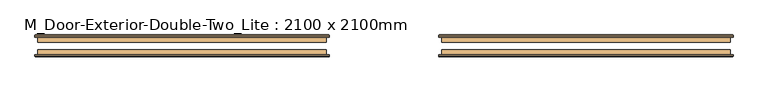
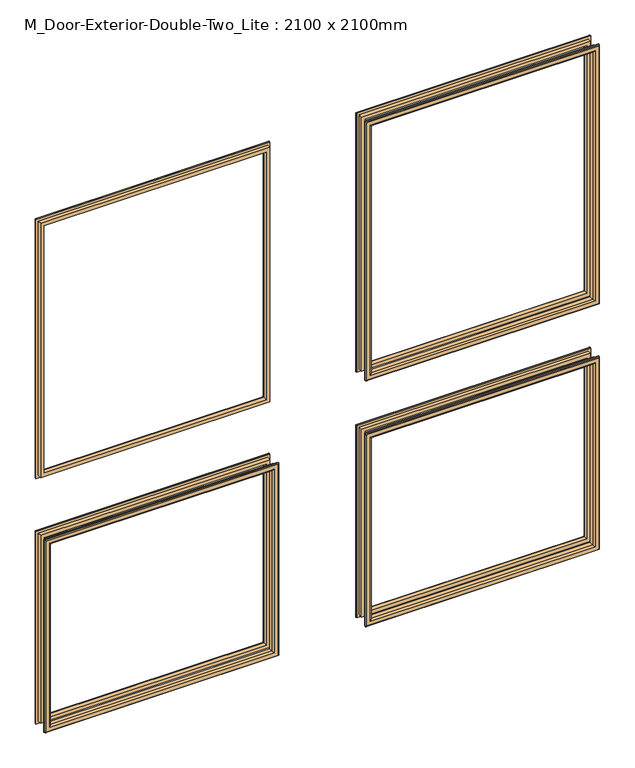
"""IFC4 building model written with IfcOpenShell, lengths in millimetres: door geometry, M_Door-Exterior-Double-Two_Lite : 2100 x 2100mm."""

from ifc_helpers import new_model, si_unit, frame, origin, place, context, project, spatial, ellipse_curve, source, transform, mapped, element, save
from ifc_brep_helpers import plane_surface, cylinder_surface, advanced_brep


def m_door_exterior_double_two_lite_2100_x_2100mm_e5180fcb(model_context):
    return source(origin(), model_context, "Body", "AdvancedBrep", [
        advanced_brep(
        [(-900.0, 31.35, 900.0), (-900.0, 43.85, 900.0), (-900.0, 43.85, 250.0), (-900.0, 31.35, 250.0), (-888.0, 44.85, 888.0), (-888.0, 31.35, 888.0), (-888.0, 31.35, 262.0), (-888.0, 44.85, 262.0), (-893.0, 49.85, 893.0), (-893.0, 49.85, 257.0), (-908.0, 47.85, 908.0), (-906.0, 49.85, 906.0), (-906.0, 49.85, 244.0), (-908.0, 47.85, 242.0), (-908.0, 43.85, 908.0), (-908.0, 43.85, 242.0), (-150.0, 43.85, 250.0), (-150.0, 31.35, 250.0), (-162.0, 31.35, 262.0), (-162.0, 44.85, 262.0), (-157.0, 49.85, 257.0), (-144.0, 49.85, 244.0), (-142.0, 47.85, 242.0), (-142.0, 43.85, 242.0), (-150.0, 43.85, 900.0), (-150.0, 31.35, 900.0), (-162.0, 31.35, 888.0), (-162.0, 44.85, 888.0), (-157.0, 49.85, 893.0), (-144.0, 49.85, 906.0), (-142.0, 47.85, 908.0), (-142.0, 43.85, 908.0)],
        [
            (0, 1),
            (1, 2),
            (2, 3),
            (3, 0),
            (4, 5),
            (5, 6),
            (6, 7),
            (7, 4),
            (8, 4, ellipse_curve(frame((-893.0, 44.85, 893.0), z_axis=(-0.7071067811865475, 0.0, -0.7071067811865475), x_axis=(-0.7071067811865474, 0.0, 0.7071067811865476)), 7.0710678, 5.0)),
            (7, 9, ellipse_curve(frame((-893.0, 44.85, 257.0), z_axis=(-0.7071067811865475, 0.0, 0.7071067811865475), x_axis=(0.7071067811865474, 0.0, 0.7071067811865476)), 7.0710678, 5.0)),
            (9, 8),
            (10, 11, ellipse_curve(frame((-906.0, 47.85, 906.0), z_axis=(-0.7071067811865475, 0.0, -0.7071067811865475), x_axis=(-0.7071067811865474, 0.0, 0.7071067811865476)), 2.8284271, 2.0)),
            (11, 12),
            (12, 13, ellipse_curve(frame((-906.0, 47.85, 244.0), z_axis=(-0.7071067811865475, 0.0, 0.7071067811865475), x_axis=(0.7071067811865474, 0.0, 0.7071067811865476)), 2.8284271, 2.0)),
            (13, 10),
            (14, 10),
            (13, 15),
            (15, 14),
            (2, 16),
            (16, 17),
            (17, 3),
            (6, 18),
            (18, 19),
            (19, 7),
            (19, 20, ellipse_curve(frame((-157.0, 44.85, 257.0), z_axis=(-0.7071067811865475, 0.0, -0.7071067811865475), x_axis=(-0.7071067811865476, 0.0, 0.7071067811865474)), 7.0710678, 5.0)),
            (20, 9),
            (12, 21),
            (21, 22, ellipse_curve(frame((-144.0, 47.85, 244.0), z_axis=(-0.7071067811865475, 0.0, -0.7071067811865475), x_axis=(-0.7071067811865476, 0.0, 0.7071067811865474)), 2.8284271, 2.0)),
            (22, 13),
            (22, 23),
            (23, 15),
            (16, 24),
            (24, 25),
            (25, 17),
            (18, 26),
            (26, 27),
            (27, 19),
            (27, 28, ellipse_curve(frame((-157.0, 44.85, 893.0), z_axis=(0.7071067811865475, 0.0, -0.7071067811865475), x_axis=(-0.7071067811865474, 0.0, -0.7071067811865476)), 7.0710678, 5.0)),
            (28, 20),
            (21, 29),
            (29, 30, ellipse_curve(frame((-144.0, 47.85, 906.0), z_axis=(0.7071067811865475, 0.0, -0.7071067811865475), x_axis=(-0.7071067811865474, 0.0, -0.7071067811865476)), 2.8284271, 2.0)),
            (30, 22),
            (30, 31),
            (31, 23),
            (31, 14),
            (1, 24),
            (0, 25),
            (5, 26),
            (4, 27),
            (8, 28),
            (11, 29),
            (10, 30),
        ],
        [
            plane_surface(frame((-900.0, 43.85, 900.0), z_axis=(-1.0, 0.0, 0.0), x_axis=(0.0, 0.0, -1.0))),
            plane_surface(frame((-888.0, 31.35, 888.0), z_axis=(1.0, 0.0, 0.0), x_axis=(0.0, 0.0, -1.0))),
            cylinder_surface(frame((-893.0, 44.85, 900.0), z_axis=(0.0, 0.0, 1.0), x_axis=(-1.0, 0.0, 0.0)), 5.0),
            cylinder_surface(frame((-906.0, 47.85, 900.0), z_axis=(0.0, 0.0, 1.0), x_axis=(-1.0, 0.0, 0.0)), 2.0),
            plane_surface(frame((-908.0, 47.85, 908.0), z_axis=(-1.0, 0.0, 0.0), x_axis=(0.0, 0.0, -1.0))),
            plane_surface(frame((-900.0, 43.85, 250.0), z_axis=(0.0, 0.0, -1.0), x_axis=(1.0, 0.0, 0.0))),
            plane_surface(frame((-888.0, 31.35, 262.0), z_axis=(0.0, 0.0, 1.0), x_axis=(1.0, 0.0, 0.0))),
            cylinder_surface(frame((-900.0, 44.85, 257.0), z_axis=(-1.0, 0.0, 0.0), x_axis=(0.0, 0.0, -1.0)), 5.0),
            cylinder_surface(frame((-900.0, 47.85, 244.0), z_axis=(-1.0, 0.0, 0.0), x_axis=(0.0, 0.0, -1.0)), 2.0),
            plane_surface(frame((-908.0, 47.85, 242.0), z_axis=(0.0, 0.0, -1.0), x_axis=(1.0, 0.0, 0.0))),
            plane_surface(frame((-150.0, 43.85, 250.0), z_axis=(1.0, 0.0, 0.0), x_axis=(0.0, 0.0, 1.0))),
            plane_surface(frame((-162.0, 31.35, 262.0), z_axis=(-1.0, 0.0, 0.0), x_axis=(0.0, 0.0, 1.0))),
            cylinder_surface(frame((-157.0, 44.85, 250.0), z_axis=(0.0, 0.0, -1.0), x_axis=(1.0, 0.0, 0.0)), 5.0),
            cylinder_surface(frame((-144.0, 47.85, 250.0), z_axis=(0.0, 0.0, -1.0), x_axis=(1.0, 0.0, 0.0)), 2.0),
            plane_surface(frame((-142.0, 47.85, 242.0), z_axis=(1.0, 0.0, 0.0), x_axis=(0.0, 0.0, 1.0))),
            plane_surface(frame((-142.0, 43.85, 908.0), z_axis=(0.0, -1.0, 0.0), x_axis=(-1.0, 0.0, 0.0))),
            plane_surface(frame((-150.0, 43.85, 900.0), z_axis=(0.0, 0.0, 1.0), x_axis=(-1.0, 0.0, 0.0))),
            plane_surface(frame((-150.0, 31.35, 900.0), z_axis=(0.0, -1.0, 0.0), x_axis=(-1.0, 0.0, 0.0))),
            plane_surface(frame((-162.0, 31.35, 888.0), z_axis=(0.0, 0.0, -1.0), x_axis=(-1.0, 0.0, 0.0))),
            cylinder_surface(frame((-150.0, 44.85, 893.0), z_axis=(1.0, 0.0, 0.0), x_axis=(0.0, 0.0, 1.0)), 5.0),
            plane_surface(frame((-157.0, 49.85, 893.0), z_axis=(0.0, 1.0, 0.0), x_axis=(-1.0, 0.0, 0.0))),
            cylinder_surface(frame((-150.0, 47.85, 906.0), z_axis=(1.0, 0.0, 0.0), x_axis=(0.0, 0.0, 1.0)), 2.0),
            plane_surface(frame((-142.0, 47.85, 908.0), z_axis=(0.0, 0.0, 1.0), x_axis=(-1.0, 0.0, 0.0))),
        ],
        [
            (0, [[1, 2, 3, 4]]),
            (1, [[5, 6, 7, 8]]),
            (2, [[9, -8, 10, 11]]),
            (3, [[12, 13, 14, 15]]),
            (4, [[16, -15, 17, 18]]),
            (5, [[-3, 19, 20, 21]]),
            (6, [[-7, 22, 23, 24]]),
            (7, [[-10, -24, 25, 26]]),
            (8, [[-14, 27, 28, 29]]),
            (9, [[-17, -29, 30, 31]]),
            (10, [[-20, 32, 33, 34]]),
            (11, [[-23, 35, 36, 37]]),
            (12, [[-25, -37, 38, 39]]),
            (13, [[-28, 40, 41, 42]]),
            (14, [[-30, -42, 43, 44]]),
            (15, [[-31, -44, 45, -18], [46, -32, -19, -2]]),
            (16, [[-33, -46, -1, 47]]),
            (17, [[-21, -34, -47, -4], [48, -35, -22, -6]]),
            (18, [[-36, -48, -5, 49]]),
            (19, [[-38, -49, -9, 50]]),
            (20, [[51, -40, -27, -13], [-26, -39, -50, -11]]),
            (21, [[-41, -51, -12, 52]]),
            (22, [[-43, -52, -16, -45]]),
        ],
    ),
        advanced_brep(
        [(150.0, 31.35, 900.0), (150.0, 43.85, 900.0), (150.0, 43.85, 250.0), (150.0, 31.35, 250.0), (162.0, 44.85, 888.0), (162.0, 31.35, 888.0), (162.0, 31.35, 262.0), (162.0, 44.85, 262.0), (157.0, 49.85, 893.0), (157.0, 49.85, 257.0), (142.0, 47.85, 908.0), (144.0, 49.85, 906.0), (144.0, 49.85, 244.0), (142.0, 47.85, 242.0), (142.0, 43.85, 908.0), (142.0, 43.85, 242.0), (900.0, 43.85, 250.0), (900.0, 31.35, 250.0), (888.0, 31.35, 262.0), (888.0, 44.85, 262.0), (893.0, 49.85, 257.0), (906.0, 49.85, 244.0), (908.0, 47.85, 242.0), (908.0, 43.85, 242.0), (900.0, 43.85, 900.0), (900.0, 31.35, 900.0), (888.0, 31.35, 888.0), (888.0, 44.85, 888.0), (893.0, 49.85, 893.0), (906.0, 49.85, 906.0), (908.0, 47.85, 908.0), (908.0, 43.85, 908.0)],
        [
            (0, 1),
            (1, 2),
            (2, 3),
            (3, 0),
            (4, 5),
            (5, 6),
            (6, 7),
            (7, 4),
            (8, 4, ellipse_curve(frame((157.0, 44.85, 893.0), z_axis=(-0.7071067811865475, 0.0, -0.7071067811865475), x_axis=(-0.7071067811865474, 0.0, 0.7071067811865476)), 7.0710678, 5.0)),
            (7, 9, ellipse_curve(frame((157.0, 44.85, 257.0), z_axis=(-0.7071067811865475, 0.0, 0.7071067811865475), x_axis=(0.7071067811865474, 0.0, 0.7071067811865476)), 7.0710678, 5.0)),
            (9, 8),
            (10, 11, ellipse_curve(frame((144.0, 47.85, 906.0), z_axis=(-0.7071067811865475, 0.0, -0.7071067811865475), x_axis=(-0.7071067811865474, 0.0, 0.7071067811865476)), 2.8284271, 2.0)),
            (11, 12),
            (12, 13, ellipse_curve(frame((144.0, 47.85, 244.0), z_axis=(-0.7071067811865475, 0.0, 0.7071067811865475), x_axis=(0.7071067811865474, 0.0, 0.7071067811865476)), 2.8284271, 2.0)),
            (13, 10),
            (14, 10),
            (13, 15),
            (15, 14),
            (2, 16),
            (16, 17),
            (17, 3),
            (6, 18),
            (18, 19),
            (19, 7),
            (19, 20, ellipse_curve(frame((893.0, 44.85, 257.0), z_axis=(-0.7071067811865475, 0.0, -0.7071067811865475), x_axis=(-0.7071067811865476, 0.0, 0.7071067811865474)), 7.0710678, 5.0)),
            (20, 9),
            (12, 21),
            (21, 22, ellipse_curve(frame((906.0, 47.85, 244.0), z_axis=(-0.7071067811865475, 0.0, -0.7071067811865475), x_axis=(-0.7071067811865476, 0.0, 0.7071067811865474)), 2.8284271, 2.0)),
            (22, 13),
            (22, 23),
            (23, 15),
            (16, 24),
            (24, 25),
            (25, 17),
            (18, 26),
            (26, 27),
            (27, 19),
            (27, 28, ellipse_curve(frame((893.0, 44.85, 893.0), z_axis=(0.7071067811865475, 0.0, -0.7071067811865475), x_axis=(-0.7071067811865474, 0.0, -0.7071067811865476)), 7.0710678, 5.0)),
            (28, 20),
            (21, 29),
            (29, 30, ellipse_curve(frame((906.0, 47.85, 906.0), z_axis=(0.7071067811865475, 0.0, -0.7071067811865475), x_axis=(-0.7071067811865474, 0.0, -0.7071067811865476)), 2.8284271, 2.0)),
            (30, 22),
            (30, 31),
            (31, 23),
            (31, 14),
            (1, 24),
            (0, 25),
            (5, 26),
            (4, 27),
            (8, 28),
            (11, 29),
            (10, 30),
        ],
        [
            plane_surface(frame((150.0, 43.85, 900.0), z_axis=(-1.0, 0.0, 0.0), x_axis=(0.0, 0.0, -1.0))),
            plane_surface(frame((162.0, 31.35, 888.0), z_axis=(1.0, 0.0, 0.0), x_axis=(0.0, 0.0, -1.0))),
            cylinder_surface(frame((157.0, 44.85, 900.0), z_axis=(0.0, 0.0, 1.0), x_axis=(-1.0, 0.0, 0.0)), 5.0),
            cylinder_surface(frame((144.0, 47.85, 900.0), z_axis=(0.0, 0.0, 1.0), x_axis=(-1.0, 0.0, 0.0)), 2.0),
            plane_surface(frame((142.0, 47.85, 908.0), z_axis=(-1.0, 0.0, 0.0), x_axis=(0.0, 0.0, -1.0))),
            plane_surface(frame((150.0, 43.85, 250.0), z_axis=(0.0, 0.0, -1.0), x_axis=(1.0, 0.0, 0.0))),
            plane_surface(frame((162.0, 31.35, 262.0), z_axis=(0.0, 0.0, 1.0), x_axis=(1.0, 0.0, 0.0))),
            cylinder_surface(frame((150.0, 44.85, 257.0), z_axis=(-1.0, 0.0, 0.0), x_axis=(0.0, 0.0, -1.0)), 5.0),
            cylinder_surface(frame((150.0, 47.85, 244.0), z_axis=(-1.0, 0.0, 0.0), x_axis=(0.0, 0.0, -1.0)), 2.0),
            plane_surface(frame((142.0, 47.85, 242.0), z_axis=(0.0, 0.0, -1.0), x_axis=(1.0, 0.0, 0.0))),
            plane_surface(frame((900.0, 43.85, 250.0), z_axis=(1.0, 0.0, 0.0), x_axis=(0.0, 0.0, 1.0))),
            plane_surface(frame((888.0, 31.35, 262.0), z_axis=(-1.0, 0.0, 0.0), x_axis=(0.0, 0.0, 1.0))),
            cylinder_surface(frame((893.0, 44.85, 250.0), z_axis=(0.0, 0.0, -1.0), x_axis=(1.0, 0.0, 0.0)), 5.0),
            cylinder_surface(frame((906.0, 47.85, 250.0), z_axis=(0.0, 0.0, -1.0), x_axis=(1.0, 0.0, 0.0)), 2.0),
            plane_surface(frame((908.0, 47.85, 242.0), z_axis=(1.0, 0.0, 0.0), x_axis=(0.0, 0.0, 1.0))),
            plane_surface(frame((908.0, 43.85, 908.0), z_axis=(0.0, -1.0, 0.0), x_axis=(-1.0, 0.0, 0.0))),
            plane_surface(frame((900.0, 43.85, 900.0), z_axis=(0.0, 0.0, 1.0), x_axis=(-1.0, 0.0, 0.0))),
            plane_surface(frame((900.0, 31.35, 900.0), z_axis=(0.0, -1.0, 0.0), x_axis=(-1.0, 0.0, 0.0))),
            plane_surface(frame((888.0, 31.35, 888.0), z_axis=(0.0, 0.0, -1.0), x_axis=(-1.0, 0.0, 0.0))),
            cylinder_surface(frame((900.0, 44.85, 893.0), z_axis=(1.0, 0.0, 0.0), x_axis=(0.0, 0.0, 1.0)), 5.0),
            plane_surface(frame((893.0, 49.85, 893.0), z_axis=(0.0, 1.0, 0.0), x_axis=(-1.0, 0.0, 0.0))),
            cylinder_surface(frame((900.0, 47.85, 906.0), z_axis=(1.0, 0.0, 0.0), x_axis=(0.0, 0.0, 1.0)), 2.0),
            plane_surface(frame((908.0, 47.85, 908.0), z_axis=(0.0, 0.0, 1.0), x_axis=(-1.0, 0.0, 0.0))),
        ],
        [
            (0, [[1, 2, 3, 4]]),
            (1, [[5, 6, 7, 8]]),
            (2, [[9, -8, 10, 11]]),
            (3, [[12, 13, 14, 15]]),
            (4, [[16, -15, 17, 18]]),
            (5, [[-3, 19, 20, 21]]),
            (6, [[-7, 22, 23, 24]]),
            (7, [[-10, -24, 25, 26]]),
            (8, [[-14, 27, 28, 29]]),
            (9, [[-17, -29, 30, 31]]),
            (10, [[-20, 32, 33, 34]]),
            (11, [[-23, 35, 36, 37]]),
            (12, [[-25, -37, 38, 39]]),
            (13, [[-28, 40, 41, 42]]),
            (14, [[-30, -42, 43, 44]]),
            (15, [[-31, -44, 45, -18], [46, -32, -19, -2]]),
            (16, [[-33, -46, -1, 47]]),
            (17, [[-21, -34, -47, -4], [48, -35, -22, -6]]),
            (18, [[-36, -48, -5, 49]]),
            (19, [[-38, -49, -9, 50]]),
            (20, [[51, -40, -27, -13], [-26, -39, -50, -11]]),
            (21, [[-41, -51, -12, 52]]),
            (22, [[-43, -52, -16, -45]]),
        ],
    ),
        advanced_brep(
        [(150.0, 31.35, 1980.0), (150.0, 43.85, 1980.0), (150.0, 43.85, 1100.0), (150.0, 31.35, 1100.0), (162.0, 44.85, 1968.0), (162.0, 31.35, 1968.0), (162.0, 31.35, 1112.0), (162.0, 44.85, 1112.0), (157.0, 49.85, 1973.0), (157.0, 49.85, 1107.0), (142.0, 47.85, 1988.0), (144.0, 49.85, 1986.0), (144.0, 49.85, 1094.0), (142.0, 47.85, 1092.0), (142.0, 43.85, 1988.0), (142.0, 43.85, 1092.0), (900.0, 43.85, 1100.0), (900.0, 31.35, 1100.0), (888.0, 31.35, 1112.0), (888.0, 44.85, 1112.0), (893.0, 49.85, 1107.0), (906.0, 49.85, 1094.0), (908.0, 47.85, 1092.0), (908.0, 43.85, 1092.0), (900.0, 43.85, 1980.0), (900.0, 31.35, 1980.0), (888.0, 31.35, 1968.0), (888.0, 44.85, 1968.0), (893.0, 49.85, 1973.0), (906.0, 49.85, 1986.0), (908.0, 47.85, 1988.0), (908.0, 43.85, 1988.0)],
        [
            (0, 1),
            (1, 2),
            (2, 3),
            (3, 0),
            (4, 5),
            (5, 6),
            (6, 7),
            (7, 4),
            (8, 4, ellipse_curve(frame((157.0, 44.85, 1973.0), z_axis=(-0.7071067811865475, 0.0, -0.7071067811865475), x_axis=(-0.7071067811865474, 0.0, 0.7071067811865476)), 7.0710678, 5.0)),
            (7, 9, ellipse_curve(frame((157.0, 44.85, 1107.0), z_axis=(-0.7071067811865475, 0.0, 0.7071067811865475), x_axis=(0.7071067811865474, 0.0, 0.7071067811865476)), 7.0710678, 5.0)),
            (9, 8),
            (10, 11, ellipse_curve(frame((144.0, 47.85, 1986.0), z_axis=(-0.7071067811865475, 0.0, -0.7071067811865475), x_axis=(-0.7071067811865474, 0.0, 0.7071067811865476)), 2.8284271, 2.0)),
            (11, 12),
            (12, 13, ellipse_curve(frame((144.0, 47.85, 1094.0), z_axis=(-0.7071067811865475, 0.0, 0.7071067811865475), x_axis=(0.7071067811865474, 0.0, 0.7071067811865476)), 2.8284271, 2.0)),
            (13, 10),
            (14, 10),
            (13, 15),
            (15, 14),
            (2, 16),
            (16, 17),
            (17, 3),
            (6, 18),
            (18, 19),
            (19, 7),
            (19, 20, ellipse_curve(frame((893.0, 44.85, 1107.0), z_axis=(-0.7071067811865475, 0.0, -0.7071067811865475), x_axis=(-0.7071067811865476, 0.0, 0.7071067811865474)), 7.0710678, 5.0)),
            (20, 9),
            (12, 21),
            (21, 22, ellipse_curve(frame((906.0, 47.85, 1094.0), z_axis=(-0.7071067811865475, 0.0, -0.7071067811865475), x_axis=(-0.7071067811865476, 0.0, 0.7071067811865474)), 2.8284271, 2.0)),
            (22, 13),
            (22, 23),
            (23, 15),
            (16, 24),
            (24, 25),
            (25, 17),
            (18, 26),
            (26, 27),
            (27, 19),
            (27, 28, ellipse_curve(frame((893.0, 44.85, 1973.0), z_axis=(0.7071067811865475, 0.0, -0.7071067811865475), x_axis=(-0.7071067811865474, 0.0, -0.7071067811865476)), 7.0710678, 5.0)),
            (28, 20),
            (21, 29),
            (29, 30, ellipse_curve(frame((906.0, 47.85, 1986.0), z_axis=(0.7071067811865475, 0.0, -0.7071067811865475), x_axis=(-0.7071067811865474, 0.0, -0.7071067811865476)), 2.8284271, 2.0)),
            (30, 22),
            (30, 31),
            (31, 23),
            (31, 14),
            (1, 24),
            (0, 25),
            (5, 26),
            (4, 27),
            (8, 28),
            (11, 29),
            (10, 30),
        ],
        [
            plane_surface(frame((150.0, 43.85, 1980.0), z_axis=(-1.0, 0.0, 0.0), x_axis=(0.0, 0.0, -1.0))),
            plane_surface(frame((162.0, 31.35, 1968.0), z_axis=(1.0, 0.0, 0.0), x_axis=(0.0, 0.0, -1.0))),
            cylinder_surface(frame((157.0, 44.85, 1980.0), z_axis=(0.0, 0.0, 1.0), x_axis=(-1.0, 0.0, 0.0)), 5.0),
            cylinder_surface(frame((144.0, 47.85, 1980.0), z_axis=(0.0, 0.0, 1.0), x_axis=(-1.0, 0.0, 0.0)), 2.0),
            plane_surface(frame((142.0, 47.85, 1988.0), z_axis=(-1.0, 0.0, 0.0), x_axis=(0.0, 0.0, -1.0))),
            plane_surface(frame((150.0, 43.85, 1100.0), z_axis=(0.0, 0.0, -1.0), x_axis=(1.0, 0.0, 0.0))),
            plane_surface(frame((162.0, 31.35, 1112.0), z_axis=(0.0, 0.0, 1.0), x_axis=(1.0, 0.0, 0.0))),
            cylinder_surface(frame((150.0, 44.85, 1107.0), z_axis=(-1.0, 0.0, 0.0), x_axis=(0.0, 0.0, -1.0)), 5.0),
            cylinder_surface(frame((150.0, 47.85, 1094.0), z_axis=(-1.0, 0.0, 0.0), x_axis=(0.0, 0.0, -1.0)), 2.0),
            plane_surface(frame((142.0, 47.85, 1092.0), z_axis=(0.0, 0.0, -1.0), x_axis=(1.0, 0.0, 0.0))),
            plane_surface(frame((900.0, 43.85, 1100.0), z_axis=(1.0, 0.0, 0.0), x_axis=(0.0, 0.0, 1.0))),
            plane_surface(frame((888.0, 31.35, 1112.0), z_axis=(-1.0, 0.0, 0.0), x_axis=(0.0, 0.0, 1.0))),
            cylinder_surface(frame((893.0, 44.85, 1100.0), z_axis=(0.0, 0.0, -1.0), x_axis=(1.0, 0.0, 0.0)), 5.0),
            cylinder_surface(frame((906.0, 47.85, 1100.0), z_axis=(0.0, 0.0, -1.0), x_axis=(1.0, 0.0, 0.0)), 2.0),
            plane_surface(frame((908.0, 47.85, 1092.0), z_axis=(1.0, 0.0, 0.0), x_axis=(0.0, 0.0, 1.0))),
            plane_surface(frame((908.0, 43.85, 1988.0), z_axis=(0.0, -1.0, 0.0), x_axis=(-1.0, 0.0, 0.0))),
            plane_surface(frame((900.0, 43.85, 1980.0), z_axis=(0.0, 0.0, 1.0), x_axis=(-1.0, 0.0, 0.0))),
            plane_surface(frame((900.0, 31.35, 1980.0), z_axis=(0.0, -1.0, 0.0), x_axis=(-1.0, 0.0, 0.0))),
            plane_surface(frame((888.0, 31.35, 1968.0), z_axis=(0.0, 0.0, -1.0), x_axis=(-1.0, 0.0, 0.0))),
            cylinder_surface(frame((900.0, 44.85, 1973.0), z_axis=(1.0, 0.0, 0.0), x_axis=(0.0, 0.0, 1.0)), 5.0),
            plane_surface(frame((893.0, 49.85, 1973.0), z_axis=(0.0, 1.0, 0.0), x_axis=(-1.0, 0.0, 0.0))),
            cylinder_surface(frame((900.0, 47.85, 1986.0), z_axis=(1.0, 0.0, 0.0), x_axis=(0.0, 0.0, 1.0)), 2.0),
            plane_surface(frame((908.0, 47.85, 1988.0), z_axis=(0.0, 0.0, 1.0), x_axis=(-1.0, 0.0, 0.0))),
        ],
        [
            (0, [[1, 2, 3, 4]]),
            (1, [[5, 6, 7, 8]]),
            (2, [[9, -8, 10, 11]]),
            (3, [[12, 13, 14, 15]]),
            (4, [[16, -15, 17, 18]]),
            (5, [[-3, 19, 20, 21]]),
            (6, [[-7, 22, 23, 24]]),
            (7, [[-10, -24, 25, 26]]),
            (8, [[-14, 27, 28, 29]]),
            (9, [[-17, -29, 30, 31]]),
            (10, [[-20, 32, 33, 34]]),
            (11, [[-23, 35, 36, 37]]),
            (12, [[-25, -37, 38, 39]]),
            (13, [[-28, 40, 41, 42]]),
            (14, [[-30, -42, 43, 44]]),
            (15, [[-31, -44, 45, -18], [46, -32, -19, -2]]),
            (16, [[-33, -46, -1, 47]]),
            (17, [[-21, -34, -47, -4], [48, -35, -22, -6]]),
            (18, [[-36, -48, -5, 49]]),
            (19, [[-38, -49, -9, 50]]),
            (20, [[51, -40, -27, -13], [-26, -39, -50, -11]]),
            (21, [[-41, -51, -12, 52]]),
            (22, [[-43, -52, -16, -45]]),
        ],
    ),
        advanced_brep(
        [(-900.0, 31.35, 1980.0), (-900.0, 43.85, 1980.0), (-900.0, 43.85, 1100.0), (-900.0, 31.35, 1100.0), (-888.0, 44.85, 1968.0), (-888.0, 31.35, 1968.0), (-888.0, 31.35, 1112.0), (-888.0, 44.85, 1112.0), (-893.0, 49.85, 1973.0), (-893.0, 49.85, 1107.0), (-908.0, 47.85, 1988.0), (-906.0, 49.85, 1986.0), (-906.0, 49.85, 1094.0), (-908.0, 47.85, 1092.0), (-908.0, 43.85, 1988.0), (-908.0, 43.85, 1092.0), (-150.0, 43.85, 1100.0), (-150.0, 31.35, 1100.0), (-162.0, 31.35, 1112.0), (-162.0, 44.85, 1112.0), (-157.0, 49.85, 1107.0), (-144.0, 49.85, 1094.0), (-142.0, 47.85, 1092.0), (-142.0, 43.85, 1092.0), (-150.0, 43.85, 1980.0), (-150.0, 31.35, 1980.0), (-162.0, 31.35, 1968.0), (-162.0, 44.85, 1968.0), (-157.0, 49.85, 1973.0), (-144.0, 49.85, 1986.0), (-142.0, 47.85, 1988.0), (-142.0, 43.85, 1988.0)],
        [
            (0, 1),
            (1, 2),
            (2, 3),
            (3, 0),
            (4, 5),
            (5, 6),
            (6, 7),
            (7, 4),
            (8, 4, ellipse_curve(frame((-893.0, 44.85, 1973.0), z_axis=(-0.7071067811865475, 0.0, -0.7071067811865475), x_axis=(-0.7071067811865474, 0.0, 0.7071067811865476)), 7.0710678, 5.0)),
            (7, 9, ellipse_curve(frame((-893.0, 44.85, 1107.0), z_axis=(-0.7071067811865475, 0.0, 0.7071067811865475), x_axis=(0.7071067811865474, 0.0, 0.7071067811865476)), 7.0710678, 5.0)),
            (9, 8),
            (10, 11, ellipse_curve(frame((-906.0, 47.85, 1986.0), z_axis=(-0.7071067811865475, 0.0, -0.7071067811865475), x_axis=(-0.7071067811865474, 0.0, 0.7071067811865476)), 2.8284271, 2.0)),
            (11, 12),
            (12, 13, ellipse_curve(frame((-906.0, 47.85, 1094.0), z_axis=(-0.7071067811865475, 0.0, 0.7071067811865475), x_axis=(0.7071067811865474, 0.0, 0.7071067811865476)), 2.8284271, 2.0)),
            (13, 10),
            (14, 10),
            (13, 15),
            (15, 14),
            (2, 16),
            (16, 17),
            (17, 3),
            (6, 18),
            (18, 19),
            (19, 7),
            (19, 20, ellipse_curve(frame((-157.0, 44.85, 1107.0), z_axis=(-0.7071067811865475, 0.0, -0.7071067811865475), x_axis=(-0.7071067811865476, 0.0, 0.7071067811865474)), 7.0710678, 5.0)),
            (20, 9),
            (12, 21),
            (21, 22, ellipse_curve(frame((-144.0, 47.85, 1094.0), z_axis=(-0.7071067811865475, 0.0, -0.7071067811865475), x_axis=(-0.7071067811865476, 0.0, 0.7071067811865474)), 2.8284271, 2.0)),
            (22, 13),
            (22, 23),
            (23, 15),
            (16, 24),
            (24, 25),
            (25, 17),
            (18, 26),
            (26, 27),
            (27, 19),
            (27, 28, ellipse_curve(frame((-157.0, 44.85, 1973.0), z_axis=(0.7071067811865475, 0.0, -0.7071067811865475), x_axis=(-0.7071067811865474, 0.0, -0.7071067811865476)), 7.0710678, 5.0)),
            (28, 20),
            (21, 29),
            (29, 30, ellipse_curve(frame((-144.0, 47.85, 1986.0), z_axis=(0.7071067811865475, 0.0, -0.7071067811865475), x_axis=(-0.7071067811865474, 0.0, -0.7071067811865476)), 2.8284271, 2.0)),
            (30, 22),
            (30, 31),
            (31, 23),
            (31, 14),
            (1, 24),
            (0, 25),
            (5, 26),
            (4, 27),
            (8, 28),
            (11, 29),
            (10, 30),
        ],
        [
            plane_surface(frame((-900.0, 43.85, 1980.0), z_axis=(-1.0, 0.0, 0.0), x_axis=(0.0, 0.0, -1.0))),
            plane_surface(frame((-888.0, 31.35, 1968.0), z_axis=(1.0, 0.0, 0.0), x_axis=(0.0, 0.0, -1.0))),
            cylinder_surface(frame((-893.0, 44.85, 1980.0), z_axis=(0.0, 0.0, 1.0), x_axis=(-1.0, 0.0, 0.0)), 5.0),
            cylinder_surface(frame((-906.0, 47.85, 1980.0), z_axis=(0.0, 0.0, 1.0), x_axis=(-1.0, 0.0, 0.0)), 2.0),
            plane_surface(frame((-908.0, 47.85, 1988.0), z_axis=(-1.0, 0.0, 0.0), x_axis=(0.0, 0.0, -1.0))),
            plane_surface(frame((-900.0, 43.85, 1100.0), z_axis=(0.0, 0.0, -1.0), x_axis=(1.0, 0.0, 0.0))),
            plane_surface(frame((-888.0, 31.35, 1112.0), z_axis=(0.0, 0.0, 1.0), x_axis=(1.0, 0.0, 0.0))),
            cylinder_surface(frame((-900.0, 44.85, 1107.0), z_axis=(-1.0, 0.0, 0.0), x_axis=(0.0, 0.0, -1.0)), 5.0),
            cylinder_surface(frame((-900.0, 47.85, 1094.0), z_axis=(-1.0, 0.0, 0.0), x_axis=(0.0, 0.0, -1.0)), 2.0),
            plane_surface(frame((-908.0, 47.85, 1092.0), z_axis=(0.0, 0.0, -1.0), x_axis=(1.0, 0.0, 0.0))),
            plane_surface(frame((-150.0, 43.85, 1100.0), z_axis=(1.0, 0.0, 0.0), x_axis=(0.0, 0.0, 1.0))),
            plane_surface(frame((-162.0, 31.35, 1112.0), z_axis=(-1.0, 0.0, 0.0), x_axis=(0.0, 0.0, 1.0))),
            cylinder_surface(frame((-157.0, 44.85, 1100.0), z_axis=(0.0, 0.0, -1.0), x_axis=(1.0, 0.0, 0.0)), 5.0),
            cylinder_surface(frame((-144.0, 47.85, 1100.0), z_axis=(0.0, 0.0, -1.0), x_axis=(1.0, 0.0, 0.0)), 2.0),
            plane_surface(frame((-142.0, 47.85, 1092.0), z_axis=(1.0, 0.0, 0.0), x_axis=(0.0, 0.0, 1.0))),
            plane_surface(frame((-142.0, 43.85, 1988.0), z_axis=(0.0, -1.0, 0.0), x_axis=(-1.0, 0.0, 0.0))),
            plane_surface(frame((-150.0, 43.85, 1980.0), z_axis=(0.0, 0.0, 1.0), x_axis=(-1.0, 0.0, 0.0))),
            plane_surface(frame((-150.0, 31.35, 1980.0), z_axis=(0.0, -1.0, 0.0), x_axis=(-1.0, 0.0, 0.0))),
            plane_surface(frame((-162.0, 31.35, 1968.0), z_axis=(0.0, 0.0, -1.0), x_axis=(-1.0, 0.0, 0.0))),
            cylinder_surface(frame((-150.0, 44.85, 1973.0), z_axis=(1.0, 0.0, 0.0), x_axis=(0.0, 0.0, 1.0)), 5.0),
            plane_surface(frame((-157.0, 49.85, 1973.0), z_axis=(0.0, 1.0, 0.0), x_axis=(-1.0, 0.0, 0.0))),
            cylinder_surface(frame((-150.0, 47.85, 1986.0), z_axis=(1.0, 0.0, 0.0), x_axis=(0.0, 0.0, 1.0)), 2.0),
            plane_surface(frame((-142.0, 47.85, 1988.0), z_axis=(0.0, 0.0, 1.0), x_axis=(-1.0, 0.0, 0.0))),
        ],
        [
            (0, [[1, 2, 3, 4]]),
            (1, [[5, 6, 7, 8]]),
            (2, [[9, -8, 10, 11]]),
            (3, [[12, 13, 14, 15]]),
            (4, [[16, -15, 17, 18]]),
            (5, [[-3, 19, 20, 21]]),
            (6, [[-7, 22, 23, 24]]),
            (7, [[-10, -24, 25, 26]]),
            (8, [[-14, 27, 28, 29]]),
            (9, [[-17, -29, 30, 31]]),
            (10, [[-20, 32, 33, 34]]),
            (11, [[-23, 35, 36, 37]]),
            (12, [[-25, -37, 38, 39]]),
            (13, [[-28, 40, 41, 42]]),
            (14, [[-30, -42, 43, 44]]),
            (15, [[-31, -44, 45, -18], [46, -32, -19, -2]]),
            (16, [[-33, -46, -1, 47]]),
            (17, [[-21, -34, -47, -4], [48, -35, -22, -6]]),
            (18, [[-36, -48, -5, 49]]),
            (19, [[-38, -49, -9, 50]]),
            (20, [[51, -40, -27, -13], [-26, -39, -50, -11]]),
            (21, [[-41, -51, -12, 52]]),
            (22, [[-43, -52, -16, -45]]),
        ],
    ),
        advanced_brep(
        [(-900.0, 11.35, 250.0), (-900.0, -1.15, 250.0), (-900.0, -1.15, 900.0), (-900.0, 11.35, 900.0), (-888.0, -2.15, 262.0), (-888.0, 11.35, 262.0), (-888.0, 11.35, 888.0), (-888.0, -2.15, 888.0), (-893.0, -7.15, 257.0), (-893.0, -7.15, 893.0), (-908.0, -5.15, 242.0), (-906.0, -7.15, 244.0), (-906.0, -7.15, 906.0), (-908.0, -5.15, 908.0), (-908.0, -1.15, 242.0), (-908.0, -1.15, 908.0), (-150.0, -1.15, 900.0), (-150.0, 11.35, 900.0), (-162.0, 11.35, 888.0), (-162.0, -2.15, 888.0), (-157.0, -7.15, 893.0), (-144.0, -7.15, 906.0), (-142.0, -5.15, 908.0), (-142.0, -1.15, 908.0), (-150.0, -1.15, 250.0), (-150.0, 11.35, 250.0), (-162.0, 11.35, 262.0), (-162.0, -2.15, 262.0), (-157.0, -7.15, 257.0), (-144.0, -7.15, 244.0), (-142.0, -5.15, 242.0), (-142.0, -1.15, 242.0)],
        [
            (0, 1),
            (1, 2),
            (2, 3),
            (3, 0),
            (4, 5),
            (5, 6),
            (6, 7),
            (7, 4),
            (8, 4, ellipse_curve(frame((-893.0, -2.15, 257.0), z_axis=(-0.7071067811865475, 0.0, 0.7071067811865475), x_axis=(-0.7071067811865474, 0.0, -0.7071067811865476)), 7.0710678, 5.0)),
            (7, 9, ellipse_curve(frame((-893.0, -2.15, 893.0), z_axis=(-0.7071067811865475, 0.0, -0.7071067811865475), x_axis=(0.7071067811865474, 0.0, -0.7071067811865476)), 7.0710678, 5.0)),
            (9, 8),
            (10, 11, ellipse_curve(frame((-906.0, -5.15, 244.0), z_axis=(-0.7071067811865475, 0.0, 0.7071067811865475), x_axis=(-0.7071067811865474, 0.0, -0.7071067811865476)), 2.8284271, 2.0)),
            (11, 12),
            (12, 13, ellipse_curve(frame((-906.0, -5.15, 906.0), z_axis=(-0.7071067811865475, 0.0, -0.7071067811865475), x_axis=(0.7071067811865474, 0.0, -0.7071067811865476)), 2.8284271, 2.0)),
            (13, 10),
            (14, 10),
            (13, 15),
            (15, 14),
            (2, 16),
            (16, 17),
            (17, 3),
            (6, 18),
            (18, 19),
            (19, 7),
            (19, 20, ellipse_curve(frame((-157.0, -2.15, 893.0), z_axis=(-0.7071067811865475, 0.0, 0.7071067811865475), x_axis=(-0.7071067811865476, 0.0, -0.7071067811865474)), 7.0710678, 5.0)),
            (20, 9),
            (12, 21),
            (21, 22, ellipse_curve(frame((-144.0, -5.15, 906.0), z_axis=(-0.7071067811865475, 0.0, 0.7071067811865475), x_axis=(-0.7071067811865476, 0.0, -0.7071067811865474)), 2.8284271, 2.0)),
            (22, 13),
            (22, 23),
            (23, 15),
            (16, 24),
            (24, 25),
            (25, 17),
            (18, 26),
            (26, 27),
            (27, 19),
            (27, 28, ellipse_curve(frame((-157.0, -2.15, 257.0), z_axis=(0.7071067811865475, 0.0, 0.7071067811865475), x_axis=(-0.7071067811865474, 0.0, 0.7071067811865476)), 7.0710678, 5.0)),
            (28, 20),
            (21, 29),
            (29, 30, ellipse_curve(frame((-144.0, -5.15, 244.0), z_axis=(0.7071067811865475, 0.0, 0.7071067811865475), x_axis=(-0.7071067811865474, 0.0, 0.7071067811865476)), 2.8284271, 2.0)),
            (30, 22),
            (30, 31),
            (31, 23),
            (31, 14),
            (1, 24),
            (0, 25),
            (5, 26),
            (4, 27),
            (8, 28),
            (11, 29),
            (10, 30),
        ],
        [
            plane_surface(frame((-900.0, -1.15, 250.0), z_axis=(-1.0, 0.0, 0.0), x_axis=(0.0, 0.0, 1.0))),
            plane_surface(frame((-888.0, 11.35, 262.0), z_axis=(1.0, 0.0, 0.0), x_axis=(0.0, 0.0, 1.0))),
            cylinder_surface(frame((-893.0, -2.15, 250.0), z_axis=(0.0, 0.0, -1.0), x_axis=(-1.0, 0.0, 0.0)), 5.0),
            cylinder_surface(frame((-906.0, -5.15, 250.0), z_axis=(0.0, 0.0, -1.0), x_axis=(-1.0, 0.0, 0.0)), 2.0),
            plane_surface(frame((-908.0, -5.15, 242.0), z_axis=(-1.0, 0.0, 0.0), x_axis=(0.0, 0.0, 1.0))),
            plane_surface(frame((-900.0, -1.15, 900.0), z_axis=(0.0, 0.0, 1.0), x_axis=(1.0, 0.0, 0.0))),
            plane_surface(frame((-888.0, 11.35, 888.0), z_axis=(0.0, 0.0, -1.0), x_axis=(1.0, 0.0, 0.0))),
            cylinder_surface(frame((-900.0, -2.15, 893.0), z_axis=(-1.0, 0.0, 0.0), x_axis=(0.0, 0.0, 1.0)), 5.0),
            cylinder_surface(frame((-900.0, -5.15, 906.0), z_axis=(-1.0, 0.0, 0.0), x_axis=(0.0, 0.0, 1.0)), 2.0),
            plane_surface(frame((-908.0, -5.15, 908.0), z_axis=(0.0, 0.0, 1.0), x_axis=(1.0, 0.0, 0.0))),
            plane_surface(frame((-150.0, -1.15, 900.0), z_axis=(1.0, 0.0, 0.0), x_axis=(0.0, 0.0, -1.0))),
            plane_surface(frame((-162.0, 11.35, 888.0), z_axis=(-1.0, 0.0, 0.0), x_axis=(0.0, 0.0, -1.0))),
            cylinder_surface(frame((-157.0, -2.15, 900.0), z_axis=(0.0, 0.0, 1.0), x_axis=(1.0, 0.0, 0.0)), 5.0),
            cylinder_surface(frame((-144.0, -5.15, 900.0), z_axis=(0.0, 0.0, 1.0), x_axis=(1.0, 0.0, 0.0)), 2.0),
            plane_surface(frame((-142.0, -5.15, 908.0), z_axis=(1.0, 0.0, 0.0), x_axis=(0.0, 0.0, -1.0))),
            plane_surface(frame((-142.0, -1.15, 242.0), z_axis=(0.0, 1.0, 0.0), x_axis=(-1.0, 0.0, 0.0))),
            plane_surface(frame((-150.0, -1.15, 250.0), z_axis=(0.0, 0.0, -1.0), x_axis=(-1.0, 0.0, 0.0))),
            plane_surface(frame((-150.0, 11.35, 250.0), z_axis=(0.0, 1.0, 0.0), x_axis=(-1.0, 0.0, 0.0))),
            plane_surface(frame((-162.0, 11.35, 262.0), z_axis=(0.0, 0.0, 1.0), x_axis=(-1.0, 0.0, 0.0))),
            cylinder_surface(frame((-150.0, -2.15, 257.0), z_axis=(1.0, 0.0, 0.0), x_axis=(0.0, 0.0, -1.0)), 5.0),
            plane_surface(frame((-157.0, -7.15, 257.0), z_axis=(0.0, -1.0, 0.0), x_axis=(-1.0, 0.0, 0.0))),
            cylinder_surface(frame((-150.0, -5.15, 244.0), z_axis=(1.0, 0.0, 0.0), x_axis=(0.0, 0.0, -1.0)), 2.0),
            plane_surface(frame((-142.0, -5.15, 242.0), z_axis=(0.0, 0.0, -1.0), x_axis=(-1.0, 0.0, 0.0))),
        ],
        [
            (0, [[1, 2, 3, 4]]),
            (1, [[5, 6, 7, 8]]),
            (2, [[9, -8, 10, 11]]),
            (3, [[12, 13, 14, 15]]),
            (4, [[16, -15, 17, 18]]),
            (5, [[-3, 19, 20, 21]]),
            (6, [[-7, 22, 23, 24]]),
            (7, [[-10, -24, 25, 26]]),
            (8, [[-14, 27, 28, 29]]),
            (9, [[-17, -29, 30, 31]]),
            (10, [[-20, 32, 33, 34]]),
            (11, [[-23, 35, 36, 37]]),
            (12, [[-25, -37, 38, 39]]),
            (13, [[-28, 40, 41, 42]]),
            (14, [[-30, -42, 43, 44]]),
            (15, [[-31, -44, 45, -18], [46, -32, -19, -2]]),
            (16, [[-33, -46, -1, 47]]),
            (17, [[-21, -34, -47, -4], [48, -35, -22, -6]]),
            (18, [[-36, -48, -5, 49]]),
            (19, [[-38, -49, -9, 50]]),
            (20, [[51, -40, -27, -13], [-26, -39, -50, -11]]),
            (21, [[-41, -51, -12, 52]]),
            (22, [[-43, -52, -16, -45]]),
        ],
    ),
        advanced_brep(
        [(150.0, 11.35, 250.0), (150.0, -1.15, 250.0), (150.0, -1.15, 900.0), (150.0, 11.35, 900.0), (162.0, -2.15, 262.0), (162.0, 11.35, 262.0), (162.0, 11.35, 888.0), (162.0, -2.15, 888.0), (157.0, -7.15, 257.0), (157.0, -7.15, 893.0), (142.0, -5.15, 242.0), (144.0, -7.15, 244.0), (144.0, -7.15, 906.0), (142.0, -5.15, 908.0), (142.0, -1.15, 242.0), (142.0, -1.15, 908.0), (900.0, -1.15, 900.0), (900.0, 11.35, 900.0), (888.0, 11.35, 888.0), (888.0, -2.15, 888.0), (893.0, -7.15, 893.0), (906.0, -7.15, 906.0), (908.0, -5.15, 908.0), (908.0, -1.15, 908.0), (900.0, -1.15, 250.0), (900.0, 11.35, 250.0), (888.0, 11.35, 262.0), (888.0, -2.15, 262.0), (893.0, -7.15, 257.0), (906.0, -7.15, 244.0), (908.0, -5.15, 242.0), (908.0, -1.15, 242.0)],
        [
            (0, 1),
            (1, 2),
            (2, 3),
            (3, 0),
            (4, 5),
            (5, 6),
            (6, 7),
            (7, 4),
            (8, 4, ellipse_curve(frame((157.0, -2.15, 257.0), z_axis=(-0.7071067811865475, 0.0, 0.7071067811865475), x_axis=(-0.7071067811865474, 0.0, -0.7071067811865476)), 7.0710678, 5.0)),
            (7, 9, ellipse_curve(frame((157.0, -2.15, 893.0), z_axis=(-0.7071067811865475, 0.0, -0.7071067811865475), x_axis=(0.7071067811865474, 0.0, -0.7071067811865476)), 7.0710678, 5.0)),
            (9, 8),
            (10, 11, ellipse_curve(frame((144.0, -5.15, 244.0), z_axis=(-0.7071067811865475, 0.0, 0.7071067811865475), x_axis=(-0.7071067811865474, 0.0, -0.7071067811865476)), 2.8284271, 2.0)),
            (11, 12),
            (12, 13, ellipse_curve(frame((144.0, -5.15, 906.0), z_axis=(-0.7071067811865475, 0.0, -0.7071067811865475), x_axis=(0.7071067811865474, 0.0, -0.7071067811865476)), 2.8284271, 2.0)),
            (13, 10),
            (14, 10),
            (13, 15),
            (15, 14),
            (2, 16),
            (16, 17),
            (17, 3),
            (6, 18),
            (18, 19),
            (19, 7),
            (19, 20, ellipse_curve(frame((893.0, -2.15, 893.0), z_axis=(-0.7071067811865475, 0.0, 0.7071067811865475), x_axis=(-0.7071067811865476, 0.0, -0.7071067811865474)), 7.0710678, 5.0)),
            (20, 9),
            (12, 21),
            (21, 22, ellipse_curve(frame((906.0, -5.15, 906.0), z_axis=(-0.7071067811865475, 0.0, 0.7071067811865475), x_axis=(-0.7071067811865476, 0.0, -0.7071067811865474)), 2.8284271, 2.0)),
            (22, 13),
            (22, 23),
            (23, 15),
            (16, 24),
            (24, 25),
            (25, 17),
            (18, 26),
            (26, 27),
            (27, 19),
            (27, 28, ellipse_curve(frame((893.0, -2.15, 257.0), z_axis=(0.7071067811865475, 0.0, 0.7071067811865475), x_axis=(-0.7071067811865474, 0.0, 0.7071067811865476)), 7.0710678, 5.0)),
            (28, 20),
            (21, 29),
            (29, 30, ellipse_curve(frame((906.0, -5.15, 244.0), z_axis=(0.7071067811865475, 0.0, 0.7071067811865475), x_axis=(-0.7071067811865474, 0.0, 0.7071067811865476)), 2.8284271, 2.0)),
            (30, 22),
            (30, 31),
            (31, 23),
            (31, 14),
            (1, 24),
            (0, 25),
            (5, 26),
            (4, 27),
            (8, 28),
            (11, 29),
            (10, 30),
        ],
        [
            plane_surface(frame((150.0, -1.15, 250.0), z_axis=(-1.0, 0.0, 0.0), x_axis=(0.0, 0.0, 1.0))),
            plane_surface(frame((162.0, 11.35, 262.0), z_axis=(1.0, 0.0, 0.0), x_axis=(0.0, 0.0, 1.0))),
            cylinder_surface(frame((157.0, -2.15, 250.0), z_axis=(0.0, 0.0, -1.0), x_axis=(-1.0, 0.0, 0.0)), 5.0),
            cylinder_surface(frame((144.0, -5.15, 250.0), z_axis=(0.0, 0.0, -1.0), x_axis=(-1.0, 0.0, 0.0)), 2.0),
            plane_surface(frame((142.0, -5.15, 242.0), z_axis=(-1.0, 0.0, 0.0), x_axis=(0.0, 0.0, 1.0))),
            plane_surface(frame((150.0, -1.15, 900.0), z_axis=(0.0, 0.0, 1.0), x_axis=(1.0, 0.0, 0.0))),
            plane_surface(frame((162.0, 11.35, 888.0), z_axis=(0.0, 0.0, -1.0), x_axis=(1.0, 0.0, 0.0))),
            cylinder_surface(frame((150.0, -2.15, 893.0), z_axis=(-1.0, 0.0, 0.0), x_axis=(0.0, 0.0, 1.0)), 5.0),
            cylinder_surface(frame((150.0, -5.15, 906.0), z_axis=(-1.0, 0.0, 0.0), x_axis=(0.0, 0.0, 1.0)), 2.0),
            plane_surface(frame((142.0, -5.15, 908.0), z_axis=(0.0, 0.0, 1.0), x_axis=(1.0, 0.0, 0.0))),
            plane_surface(frame((900.0, -1.15, 900.0), z_axis=(1.0, 0.0, 0.0), x_axis=(0.0, 0.0, -1.0))),
            plane_surface(frame((888.0, 11.35, 888.0), z_axis=(-1.0, 0.0, 0.0), x_axis=(0.0, 0.0, -1.0))),
            cylinder_surface(frame((893.0, -2.15, 900.0), z_axis=(0.0, 0.0, 1.0), x_axis=(1.0, 0.0, 0.0)), 5.0),
            cylinder_surface(frame((906.0, -5.15, 900.0), z_axis=(0.0, 0.0, 1.0), x_axis=(1.0, 0.0, 0.0)), 2.0),
            plane_surface(frame((908.0, -5.15, 908.0), z_axis=(1.0, 0.0, 0.0), x_axis=(0.0, 0.0, -1.0))),
            plane_surface(frame((908.0, -1.15, 242.0), z_axis=(0.0, 1.0, 0.0), x_axis=(-1.0, 0.0, 0.0))),
            plane_surface(frame((900.0, -1.15, 250.0), z_axis=(0.0, 0.0, -1.0), x_axis=(-1.0, 0.0, 0.0))),
            plane_surface(frame((900.0, 11.35, 250.0), z_axis=(0.0, 1.0, 0.0), x_axis=(-1.0, 0.0, 0.0))),
            plane_surface(frame((888.0, 11.35, 262.0), z_axis=(0.0, 0.0, 1.0), x_axis=(-1.0, 0.0, 0.0))),
            cylinder_surface(frame((900.0, -2.15, 257.0), z_axis=(1.0, 0.0, 0.0), x_axis=(0.0, 0.0, -1.0)), 5.0),
            plane_surface(frame((893.0, -7.15, 257.0), z_axis=(0.0, -1.0, 0.0), x_axis=(-1.0, 0.0, 0.0))),
            cylinder_surface(frame((900.0, -5.15, 244.0), z_axis=(1.0, 0.0, 0.0), x_axis=(0.0, 0.0, -1.0)), 2.0),
            plane_surface(frame((908.0, -5.15, 242.0), z_axis=(0.0, 0.0, -1.0), x_axis=(-1.0, 0.0, 0.0))),
        ],
        [
            (0, [[1, 2, 3, 4]]),
            (1, [[5, 6, 7, 8]]),
            (2, [[9, -8, 10, 11]]),
            (3, [[12, 13, 14, 15]]),
            (4, [[16, -15, 17, 18]]),
            (5, [[-3, 19, 20, 21]]),
            (6, [[-7, 22, 23, 24]]),
            (7, [[-10, -24, 25, 26]]),
            (8, [[-14, 27, 28, 29]]),
            (9, [[-17, -29, 30, 31]]),
            (10, [[-20, 32, 33, 34]]),
            (11, [[-23, 35, 36, 37]]),
            (12, [[-25, -37, 38, 39]]),
            (13, [[-28, 40, 41, 42]]),
            (14, [[-30, -42, 43, 44]]),
            (15, [[-31, -44, 45, -18], [46, -32, -19, -2]]),
            (16, [[-33, -46, -1, 47]]),
            (17, [[-21, -34, -47, -4], [48, -35, -22, -6]]),
            (18, [[-36, -48, -5, 49]]),
            (19, [[-38, -49, -9, 50]]),
            (20, [[51, -40, -27, -13], [-26, -39, -50, -11]]),
            (21, [[-41, -51, -12, 52]]),
            (22, [[-43, -52, -16, -45]]),
        ],
    ),
        advanced_brep(
        [(150.0, 11.35, 1100.0), (150.0, -1.15, 1100.0), (150.0, -1.15, 1980.0), (150.0, 11.35, 1980.0), (162.0, -2.15, 1112.0), (162.0, 11.35, 1112.0), (162.0, 11.35, 1968.0), (162.0, -2.15, 1968.0), (157.0, -7.15, 1107.0), (157.0, -7.15, 1973.0), (142.0, -5.15, 1092.0), (144.0, -7.15, 1094.0), (144.0, -7.15, 1986.0), (142.0, -5.15, 1988.0), (142.0, -1.15, 1092.0), (142.0, -1.15, 1988.0), (900.0, -1.15, 1980.0), (900.0, 11.35, 1980.0), (888.0, 11.35, 1968.0), (888.0, -2.15, 1968.0), (893.0, -7.15, 1973.0), (906.0, -7.15, 1986.0), (908.0, -5.15, 1988.0), (908.0, -1.15, 1988.0), (900.0, -1.15, 1100.0), (900.0, 11.35, 1100.0), (888.0, 11.35, 1112.0), (888.0, -2.15, 1112.0), (893.0, -7.15, 1107.0), (906.0, -7.15, 1094.0), (908.0, -5.15, 1092.0), (908.0, -1.15, 1092.0)],
        [
            (0, 1),
            (1, 2),
            (2, 3),
            (3, 0),
            (4, 5),
            (5, 6),
            (6, 7),
            (7, 4),
            (8, 4, ellipse_curve(frame((157.0, -2.15, 1107.0), z_axis=(-0.7071067811865475, 0.0, 0.7071067811865475), x_axis=(-0.7071067811865474, 0.0, -0.7071067811865476)), 7.0710678, 5.0)),
            (7, 9, ellipse_curve(frame((157.0, -2.15, 1973.0), z_axis=(-0.7071067811865475, 0.0, -0.7071067811865475), x_axis=(0.7071067811865474, 0.0, -0.7071067811865476)), 7.0710678, 5.0)),
            (9, 8),
            (10, 11, ellipse_curve(frame((144.0, -5.15, 1094.0), z_axis=(-0.7071067811865475, 0.0, 0.7071067811865475), x_axis=(-0.7071067811865474, 0.0, -0.7071067811865476)), 2.8284271, 2.0)),
            (11, 12),
            (12, 13, ellipse_curve(frame((144.0, -5.15, 1986.0), z_axis=(-0.7071067811865475, 0.0, -0.7071067811865475), x_axis=(0.7071067811865474, 0.0, -0.7071067811865476)), 2.8284271, 2.0)),
            (13, 10),
            (14, 10),
            (13, 15),
            (15, 14),
            (2, 16),
            (16, 17),
            (17, 3),
            (6, 18),
            (18, 19),
            (19, 7),
            (19, 20, ellipse_curve(frame((893.0, -2.15, 1973.0), z_axis=(-0.7071067811865475, 0.0, 0.7071067811865475), x_axis=(-0.7071067811865476, 0.0, -0.7071067811865474)), 7.0710678, 5.0)),
            (20, 9),
            (12, 21),
            (21, 22, ellipse_curve(frame((906.0, -5.15, 1986.0), z_axis=(-0.7071067811865475, 0.0, 0.7071067811865475), x_axis=(-0.7071067811865476, 0.0, -0.7071067811865474)), 2.8284271, 2.0)),
            (22, 13),
            (22, 23),
            (23, 15),
            (16, 24),
            (24, 25),
            (25, 17),
            (18, 26),
            (26, 27),
            (27, 19),
            (27, 28, ellipse_curve(frame((893.0, -2.15, 1107.0), z_axis=(0.7071067811865475, 0.0, 0.7071067811865475), x_axis=(-0.7071067811865474, 0.0, 0.7071067811865476)), 7.0710678, 5.0)),
            (28, 20),
            (21, 29),
            (29, 30, ellipse_curve(frame((906.0, -5.15, 1094.0), z_axis=(0.7071067811865475, 0.0, 0.7071067811865475), x_axis=(-0.7071067811865474, 0.0, 0.7071067811865476)), 2.8284271, 2.0)),
            (30, 22),
            (30, 31),
            (31, 23),
            (31, 14),
            (1, 24),
            (0, 25),
            (5, 26),
            (4, 27),
            (8, 28),
            (11, 29),
            (10, 30),
        ],
        [
            plane_surface(frame((150.0, -1.15, 1100.0), z_axis=(-1.0, 0.0, 0.0), x_axis=(0.0, 0.0, 1.0))),
            plane_surface(frame((162.0, 11.35, 1112.0), z_axis=(1.0, 0.0, 0.0), x_axis=(0.0, 0.0, 1.0))),
            cylinder_surface(frame((157.0, -2.15, 1100.0), z_axis=(0.0, 0.0, -1.0), x_axis=(-1.0, 0.0, 0.0)), 5.0),
            cylinder_surface(frame((144.0, -5.15, 1100.0), z_axis=(0.0, 0.0, -1.0), x_axis=(-1.0, 0.0, 0.0)), 2.0),
            plane_surface(frame((142.0, -5.15, 1092.0), z_axis=(-1.0, 0.0, 0.0), x_axis=(0.0, 0.0, 1.0))),
            plane_surface(frame((150.0, -1.15, 1980.0), z_axis=(0.0, 0.0, 1.0), x_axis=(1.0, 0.0, 0.0))),
            plane_surface(frame((162.0, 11.35, 1968.0), z_axis=(0.0, 0.0, -1.0), x_axis=(1.0, 0.0, 0.0))),
            cylinder_surface(frame((150.0, -2.15, 1973.0), z_axis=(-1.0, 0.0, 0.0), x_axis=(0.0, 0.0, 1.0)), 5.0),
            cylinder_surface(frame((150.0, -5.15, 1986.0), z_axis=(-1.0, 0.0, 0.0), x_axis=(0.0, 0.0, 1.0)), 2.0),
            plane_surface(frame((142.0, -5.15, 1988.0), z_axis=(0.0, 0.0, 1.0), x_axis=(1.0, 0.0, 0.0))),
            plane_surface(frame((900.0, -1.15, 1980.0), z_axis=(1.0, 0.0, 0.0), x_axis=(0.0, 0.0, -1.0))),
            plane_surface(frame((888.0, 11.35, 1968.0), z_axis=(-1.0, 0.0, 0.0), x_axis=(0.0, 0.0, -1.0))),
            cylinder_surface(frame((893.0, -2.15, 1980.0), z_axis=(0.0, 0.0, 1.0), x_axis=(1.0, 0.0, 0.0)), 5.0),
            cylinder_surface(frame((906.0, -5.15, 1980.0), z_axis=(0.0, 0.0, 1.0), x_axis=(1.0, 0.0, 0.0)), 2.0),
            plane_surface(frame((908.0, -5.15, 1988.0), z_axis=(1.0, 0.0, 0.0), x_axis=(0.0, 0.0, -1.0))),
            plane_surface(frame((908.0, -1.15, 1092.0), z_axis=(0.0, 1.0, 0.0), x_axis=(-1.0, 0.0, 0.0))),
            plane_surface(frame((900.0, -1.15, 1100.0), z_axis=(0.0, 0.0, -1.0), x_axis=(-1.0, 0.0, 0.0))),
            plane_surface(frame((900.0, 11.35, 1100.0), z_axis=(0.0, 1.0, 0.0), x_axis=(-1.0, 0.0, 0.0))),
            plane_surface(frame((888.0, 11.35, 1112.0), z_axis=(0.0, 0.0, 1.0), x_axis=(-1.0, 0.0, 0.0))),
            cylinder_surface(frame((900.0, -2.15, 1107.0), z_axis=(1.0, 0.0, 0.0), x_axis=(0.0, 0.0, -1.0)), 5.0),
            plane_surface(frame((893.0, -7.15, 1107.0), z_axis=(0.0, -1.0, 0.0), x_axis=(-1.0, 0.0, 0.0))),
            cylinder_surface(frame((900.0, -5.15, 1094.0), z_axis=(1.0, 0.0, 0.0), x_axis=(0.0, 0.0, -1.0)), 2.0),
            plane_surface(frame((908.0, -5.15, 1092.0), z_axis=(0.0, 0.0, -1.0), x_axis=(-1.0, 0.0, 0.0))),
        ],
        [
            (0, [[1, 2, 3, 4]]),
            (1, [[5, 6, 7, 8]]),
            (2, [[9, -8, 10, 11]]),
            (3, [[12, 13, 14, 15]]),
            (4, [[16, -15, 17, 18]]),
            (5, [[-3, 19, 20, 21]]),
            (6, [[-7, 22, 23, 24]]),
            (7, [[-10, -24, 25, 26]]),
            (8, [[-14, 27, 28, 29]]),
            (9, [[-17, -29, 30, 31]]),
            (10, [[-20, 32, 33, 34]]),
            (11, [[-23, 35, 36, 37]]),
            (12, [[-25, -37, 38, 39]]),
            (13, [[-28, 40, 41, 42]]),
            (14, [[-30, -42, 43, 44]]),
            (15, [[-31, -44, 45, -18], [46, -32, -19, -2]]),
            (16, [[-33, -46, -1, 47]]),
            (17, [[-21, -34, -47, -4], [48, -35, -22, -6]]),
            (18, [[-36, -48, -5, 49]]),
            (19, [[-38, -49, -9, 50]]),
            (20, [[51, -40, -27, -13], [-26, -39, -50, -11]]),
            (21, [[-41, -51, -12, 52]]),
            (22, [[-43, -52, -16, -45]]),
        ],
    ),
    ])


if __name__ == "__main__":
    model = new_model("IFC4")
    model_context = context("Model", 3, world=origin())
    ifc_project = project(units=[si_unit("LENGTHUNIT", "METRE", prefix="MILLI")], contexts=[model_context])
    site = spatial("IfcSite", under=ifc_project)
    building = spatial("IfcBuilding", under=site)
    placement = place(None, origin())
    m_door_exterior_double_two_lite_2100_x_2100mm_shape = m_door_exterior_double_two_lite_2100_x_2100mm_e5180fcb(model_context)
    element("IfcDoor", 1, ObjectType="M_Door-Exterior-Double-Two_Lite : 2100 x 2100mm", at=placement, inside=building, context=model_context, shape_type="MappedRepresentation", body=[
        mapped(m_door_exterior_double_two_lite_2100_x_2100mm_shape, transform((0.0, 0.0, 0.0), x_axis=(1.0, 0.0, 0.0), y_axis=(0.0, 1.0, 0.0), z_axis=(0.0, 0.0, 1.0))),
    ])
    save(model, "model.ifc")

# Revit data of these elements
# Type "M_Door-Exterior-Double-Two_Lite : 2100 x 2100mm"
#   Type Mark = "46"
#   Assembly Code = "B2030100"
#   Analytic Construction = "Metal frame, double glass door"
#   Top Rail = 120 mm
#   Threshold Length [instance default] = 2200 mm
#   Threshold Offset [instance default] = 15 mm
#   Thickness = 45 mm
#   Thermal Resistance (R) = 0.242926 (m²·K)/W
#   Swing Angle [instance default] = 90.00°
#   Strike Height = 1000 mm
#   Stiles = 150 mm
#   SinglePanelWidth = 1050 mm
#   Rough Width [instance default] = 2200 mm
#   Rough Height [instance default] = 2200 mm
#   MFOpeningHeight [instance default] = 100 mm
#   MFOpeningWidth [instance default] = 100 mm
#   Lock Rail = 200 mm
#   Inset Calculate [instance default] = 105 mm
#   Masonry Inset [instance default] = 25 mm
#   Height = 2100 mm
#   Width = 2100 mm
#   Heat Transfer Coefficient (U) = 4.11674 W/(m²·K)
#   Glass Thickness = 20 mm
#   Masonry Frame Depth = 150 mm
#   Bottom Rail = 250 mm
#   Threshold [instance default] = yes
#   Masonry Frame [instance default] = yes
#   Function = 1
#   Dry Wall Frame [instance default] = no
#   Threshold Material = Cherry
#   Panic Bar Material = Metal - Stainless Steel
#   Panel Material = Metal - Painted - Grey
#   Glass Stop Material = Metal - Painted - Grey
#   Frame Material = Metal - Painted - Grey
#   Exterior Pull Material = Metal - Stainless Steel
#   Visual Light Transmittance = 0
#   Solar Heat Gain Coefficient = 0
#   Wall Closure = (empty or 0)
# Element 1 (IfcDoor, "M_Door-Exterior-Double-Two_Lite : 2100 x 2100mm")
#   Materials on its faces: "Metal - Painted - Grey", "Metal - Stainless Steel", "Glass", "Cherry"
# Materials
#   "Cherry": class "Wood", colour RGB 226 177 128, transparency 0, Description = "Prunus Serotina", Cost = 0
#   "Metal - Stainless Steel": class "Metal", colour RGB 247 247 247, transparency 0
#   "Metal - Painted - Grey": class "Paint", colour RGB 104 104 104, transparency 0, Cost = 0
#   "Glass": class "Glass", colour RGB 0 128 192, transparency 0.9, Description = "Soda Lime Glass", Cost = 0
